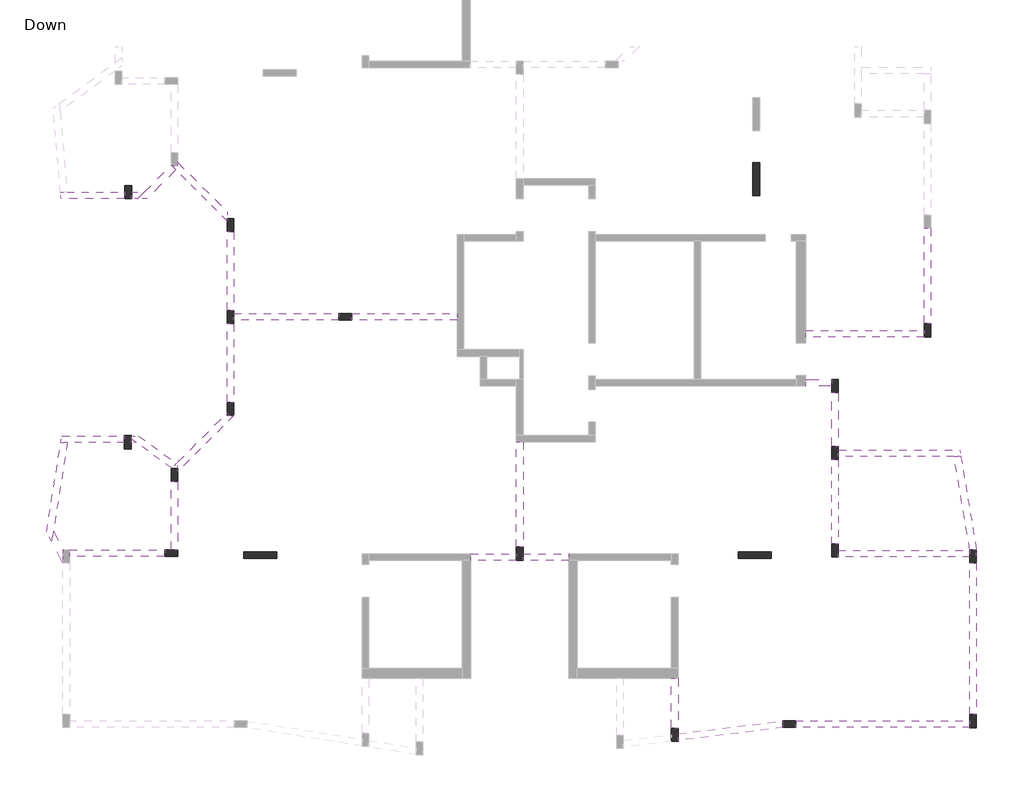
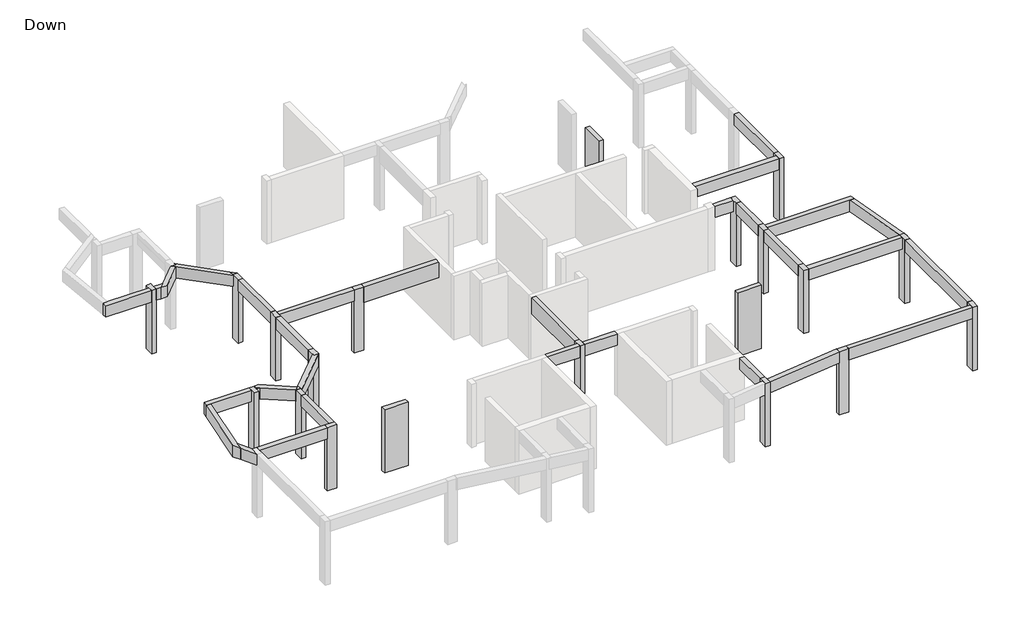
# One storey, part 2 of 3: 31 beams, 20 columns.
"""IFC4 building model written with IfcOpenShell, lengths in millimetres."""

from ifc_helpers import new_model, si_unit, frame, origin, origin_with_axes, place, context, project, spatial, polyline, outline, extrude, faceted_brep, element, save

model = new_model("IFC4")

# Units and contexts
model_context = context("Model", 3, world=origin())
ifc_project = project(units=[si_unit("LENGTHUNIT", "METRE", prefix="MILLI")], contexts=[model_context])

# Site, building, storey
site = spatial("IfcSite", under=ifc_project)
building = spatial("IfcBuilding", under=site)
storey = spatial("IfcBuildingStorey", under=building, Name="Down", Elevation=0.0)

# Beams
placement = place(None, origin())
element("IfcBeam", 1, ObjectType="Concrete Rectengular Beam : 20/50", at=placement, inside=storey, context=model_context, shape_type="Brep", body=[
    faceted_brep([(-18379.347479, -11765.3513235, 2850.0), (-18379.347479, -11965.3513235, 2850.0), (-15486.5645409, -11965.3513235, 2850.0), (-15486.5645409, -11765.3513235, 2850.0), (-18379.347479, -11965.3513235, 2650.0), (-18379.347479, -11965.3513235, 2350.0), (-15486.5645409, -11965.3513235, 2350.0), (-15486.5645409, -11965.3513235, 2650.0), (-18379.347479, -11765.3513235, 2350.0), (-15486.5645409, -11765.3513235, 2350.0)], [[[0, 1, 2, 3]], [[2, 1, 4, 5, 6, 7]], [[5, 8, 9, 6]], [[8, 0, 3, 9]], [[1, 0, 8, 5, 4]], [[3, 2, 7, 6, 9]]]),
])
element("IfcBeam", 2, ObjectType="Concrete Rectengular Beam : 20/50", at=placement, inside=storey, context=model_context, shape_type="Brep", body=[
    faceted_brep([(-15286.5645409, -9691.9014804, 2850.0), (-15286.5645409, -11765.3513235, 2850.0), (-15089.2187138, -11765.3513235, 2850.0), (-15089.2187138, -9691.9014804, 2850.0), (-15286.5645409, -11765.3513235, 2350.0), (-15286.5645409, -11765.3513235, 2650.0), (-15286.5645409, -9691.9014804, 2350.0), (-15086.5645409, -9691.9014804, 2350.0), (-15086.5645409, -11765.3513235, 2350.0), (-15086.5645409, -9691.9014804, 2650.0), (-15086.5645409, -11765.3513235, 2650.0), (-15089.2187138, -9691.9014804, 2650.0), (-15089.2187138, -11765.3513235, 2650.0)], [[[0, 1, 2, 3]], [[4, 5, 1, 0, 6]], [[6, 7, 8, 4]], [[8, 7, 9, 10]], [[7, 6, 0, 3, 11, 9]], [[1, 5, 4, 8, 10, 12, 2]], [[11, 12, 10, 9]], [[12, 11, 3, 2]]]),
    faceted_brep([(-15086.5645409, -9098.1046694, 2850.0), (-15086.5645409, -9098.1046694, 2350.0), (-15129.6352736, -9141.1754021, 2350.0), (-15272.8194649, -9284.3595934, 2350.0), (-15280.3613519, -9291.9014804, 2350.0), (-15280.3613519, -9291.9014804, 2850.0), (-15272.8194649, -9284.3595934, 2850.0), (-15129.6352736, -9141.1754021, 2850.0), (-15086.5645409, -9291.9014804, 2850.0), (-15086.5645409, -9291.9014804, 2350.0)], [[[0, 1, 2, 3, 4, 5, 6, 7]], [[8, 5, 4, 9]], [[5, 8, 0, 7, 6]], [[9, 4, 3, 2, 1]], [[1, 0, 8, 9]]]),
])
element("IfcBeam", 3, ObjectType="Concrete Rectengular Beam : 20/50", at=placement, inside=storey, context=model_context, shape_type="Brep", body=[
    faceted_brep([(-13387.4363964, -7681.8192373, 2850.0), (-13587.4363964, -7681.8192373, 2850.0), (-13587.4363964, -7598.9765249, 2850.0), (-15086.5645409, -9098.1046694, 2850.0), (-15086.5645409, -9291.9014804, 2850.0), (-15086.5645409, -9380.9473819, 2850.0), (-15086.5645409, -9380.9473819, 2650.0), (-15086.5645409, -9380.9473819, 2350.0), (-13387.4363964, -7681.8192373, 2350.0), (-13387.4363964, -7681.8192373, 2650.0), (-13587.4363964, -7681.8192373, 2350.0), (-15086.5645409, -9291.9014804, 2350.0), (-15086.5645409, -9098.1046694, 2350.0), (-13587.4363964, -7598.9765249, 2350.0)], [[[0, 1, 2, 3, 4, 5]], [[0, 5, 6, 7, 8, 9]], [[10, 8, 7, 11, 12, 13]], [[2, 13, 12, 3]], [[10, 1, 0, 9, 8]], [[1, 10, 13, 2]], [[3, 12, 11, 7, 6, 5, 4]]]),
])
element("IfcBeam", 4, ObjectType="Concrete Rectengular Beam : 20/50", at=placement, inside=storey, context=model_context, shape_type="Brep", body=[
    faceted_brep([(-15272.8194649, -9284.3595934, 2850.0), (-15129.6352736, -9141.1754021, 2850.0), (-16288.4232212, -8299.2666773, 2850.0), (-16461.5111803, -8299.2666773, 2850.0), (-16508.8112897, -8364.3696928, 2850.0), (-16508.8112897, -8386.3589683, 2850.0), (-16353.4071605, -8499.2666773, 2850.0), (-15286.5645409, -9274.373211, 2850.0), (-15129.6352736, -9141.1754021, 2350.0), (-16288.4232212, -8299.2666773, 2350.0), (-15272.8194649, -9284.3595934, 2350.0), (-16353.4071605, -8499.2666773, 2350.0), (-16508.8112897, -8386.3589683, 2350.0), (-16508.8112897, -8364.3696928, 2350.0), (-16461.5111803, -8299.2666773, 2350.0)], [[[0, 1, 2, 3, 4, 5, 6, 7]], [[1, 8, 9, 2]], [[8, 10, 11, 12, 13, 14, 9]], [[5, 12, 11, 10, 0, 7, 6]], [[1, 0, 10, 8]], [[3, 14, 13, 4]], [[3, 2, 9, 14]], [[5, 4, 13, 12]]]),
])
element("IfcBeam", 5, ObjectType="Concrete Rectengular Beam : 20/50", at=placement, inside=storey, context=model_context, shape_type="Brep", body=[
    faceted_brep([(-16508.8112897, -8386.3589683, 2850.0), (-16508.8112897, -8499.2666773, 2850.0), (-16353.4071605, -8499.2666773, 2850.0), (-16508.8112897, -8499.2666773, 2650.0), (-16508.8112897, -8499.2666773, 2350.0), (-16353.4071605, -8499.2666773, 2350.0), (-16353.4071605, -8499.2666773, 2650.0), (-16508.8112897, -8386.3589683, 2350.0)], [[[0, 1, 2]], [[1, 3, 4, 5, 6, 2]], [[4, 3, 1, 0, 7]], [[0, 2, 6, 5, 7]], [[4, 7, 5]]]),
    faceted_brep([(-16508.8112897, -8299.2666773, 2350.0), (-16508.8112897, -8299.2666773, 2850.0), (-16461.5111803, -8299.2666773, 2850.0), (-16461.5111803, -8299.2666773, 2350.0), (-16508.8112897, -8364.3696928, 2350.0), (-16508.8112897, -8364.3696928, 2850.0)], [[[0, 1, 2, 3]], [[4, 0, 3]], [[2, 5, 4, 3]], [[1, 5, 2]], [[1, 0, 4, 5]]]),
])
element("IfcBeam", 6, ObjectType="Concrete Rectengular Beam : 20/50", at=placement, inside=storey, context=model_context, shape_type="Brep", body=[
    faceted_brep([(-16708.8112897, -8499.2666773, 2850.0), (-16708.8112897, -8299.2666773, 2850.0), (-18614.2193583, -8299.2666773, 2850.0), (-18645.8962463, -8499.2666773, 2850.0), (-18443.4032212, -8499.2666773, 2850.0), (-16708.8112897, -8299.2666773, 2350.0), (-18614.2193583, -8299.2666773, 2350.0), (-16708.8112897, -8499.2666773, 2350.0), (-18443.4032212, -8499.2666773, 2350.0), (-18645.8962463, -8499.2666773, 2350.0), (-16708.8112897, -8499.2666773, 2650.0)], [[[0, 1, 2, 3, 4]], [[1, 5, 6, 2]], [[5, 7, 8, 9, 6]], [[7, 10, 0, 4, 3, 9, 8]], [[1, 0, 10, 7, 5]], [[3, 2, 6, 9]]]),
])
element("IfcBeam", 7, ObjectType="Concrete Rectengular Beam : 20/50", at=placement, inside=storey, context=model_context, shape_type="Brep", body=[
    faceted_brep([(-18443.4032212, -8499.2666773, 2850.0), (-18645.8962463, -8499.2666773, 2850.0), (-19077.0882285, -11221.7057077, 2850.0), (-18921.0696697, -11515.1339402, 2850.0), (-18869.0821124, -11186.8974215, 2850.0), (-18645.8962463, -8499.2666773, 2350.0), (-19077.0882285, -11221.7057077, 2350.0), (-18443.4032212, -8499.2666773, 2350.0), (-18869.0821124, -11186.8974215, 2350.0), (-18921.0696697, -11515.1339402, 2350.0), (-18443.4032212, -8499.2666773, 2650.0)], [[[0, 1, 2, 3, 4]], [[1, 5, 6, 2]], [[5, 7, 8, 9, 6]], [[3, 9, 8, 7, 10, 0, 4]], [[1, 0, 10, 7, 5]], [[3, 2, 6, 9]]]),
])
element("IfcBeam", 8, ObjectType="Concrete Rectengular Beam : 20/50", at=placement, inside=storey, context=model_context, shape_type="Brep", body=[
    faceted_brep([(-18869.0821124, -11186.8974215, 2850.0), (-18561.5127169, -11765.3513235, 2850.0), (-18561.5127169, -11765.3513235, 2650.0), (-18561.5127169, -11765.3513235, 2350.0), (-18869.0821124, -11186.8974215, 2350.0), (-18869.0821124, -11186.8974215, 2650.0), (-18921.0696697, -11515.1339402, 2850.0), (-18921.0696697, -11515.1339402, 2350.0), (-18579.347479, -11765.3513235, 2350.0), (-18579.347479, -11765.3513235, 2850.0), (-18579.347479, -11965.3513235, 2850.0), (-18579.347479, -12157.819908, 2850.0), (-18579.347479, -12157.819908, 2350.0), (-18579.347479, -11965.3513235, 2350.0)], [[[0, 1, 2, 3, 4, 5]], [[6, 0, 5, 4, 7]], [[8, 9, 10, 11, 12, 13]], [[9, 8, 3, 2, 1]], [[0, 6, 11, 10, 9, 1]], [[6, 7, 12, 11]], [[7, 4, 3, 8, 13, 12]]]),
])
element("IfcBeam", 9, ObjectType="Concrete Rectengular Beam : 20/50", at=placement, inside=storey, context=model_context, shape_type="Brep", body=[
    faceted_brep([(-13387.4363964, -4887.4320305, 2850.0), (-13587.4363964, -4887.4320305, 2850.0), (-13587.4363964, -7281.8192373, 2850.0), (-13387.4363964, -7281.8192373, 2850.0), (-13387.4363964, -7281.8192373, 2650.0), (-13387.4363964, -7281.8192373, 2350.0), (-13387.4363964, -4887.4320305, 2350.0), (-13387.4363964, -4887.4320305, 2650.0), (-13587.4363964, -4887.4320305, 2350.0), (-13587.4363964, -7281.8192373, 2350.0)], [[[0, 1, 2, 3]], [[0, 3, 4, 5, 6, 7]], [[8, 6, 5, 9]], [[1, 8, 9, 2]], [[1, 0, 7, 6, 8]], [[3, 2, 9, 5, 4]]]),
])
element("IfcBeam", 10, ObjectType="Concrete Rectengular Beam : 20/50", at=placement, inside=storey, context=model_context, shape_type="Brep", body=[
    faceted_brep([(-13387.4363964, -4587.4320305, 2850.0), (-13387.4363964, -4787.4320305, 2850.0), (-10195.9008278, -4787.4320305, 2850.0), (-10195.9008278, -4587.4320305, 2850.0), (-13387.4363964, -4787.4320305, 2650.0), (-13387.4363964, -4787.4320305, 2350.0), (-10195.9008278, -4787.4320305, 2350.0), (-13387.4363964, -4587.4320305, 2350.0), (-10195.9008278, -4587.4320305, 2350.0), (-13387.4363964, -4587.4320305, 2650.0)], [[[0, 1, 2, 3]], [[1, 4, 5, 6, 2]], [[5, 7, 8, 6]], [[7, 9, 0, 3, 8]], [[5, 4, 1, 0, 9, 7]], [[3, 2, 6, 8]]]),
])
element("IfcBeam", 11, ObjectType="Concrete Rectengular Beam : 20/50", at=placement, inside=storey, context=model_context, shape_type="Brep", body=[
    faceted_brep([(-13387.4363964, -2088.5879682, 2850.0), (-13587.4363964, -2088.5879682, 2850.0), (-13587.4363964, -4487.4320305, 2850.0), (-13387.4363964, -4487.4320305, 2850.0), (-13387.4363964, -4487.4320305, 2650.0), (-13387.4363964, -4487.4320305, 2350.0), (-13387.4363964, -2088.5879682, 2350.0), (-13387.4363964, -2088.5879682, 2650.0), (-13587.4363964, -2088.5879682, 2350.0), (-13587.4363964, -4487.4320305, 2350.0)], [[[0, 1, 2, 3]], [[0, 3, 4, 5, 6, 7]], [[8, 6, 5, 9]], [[1, 8, 9, 2]], [[1, 0, 7, 6, 8]], [[3, 2, 9, 5, 4]]]),
    faceted_brep([(-13387.4363964, -1685.7442295, 2350.0), (-13587.4363964, -1485.8326961, 2350.0), (-13587.4363964, -1485.8326961, 2650.0), (-13387.4363964, -1685.7442295, 2650.0), (-13587.4363964, -1688.5879682, 2350.0), (-13387.4363964, -1688.5879682, 2350.0), (-13387.4363964, -1688.5879682, 2650.0), (-13388.8740156, -1688.5879682, 2650.0), (-13388.8740156, -1688.5879682, 2850.0), (-13587.4363964, -1688.5879682, 2850.0), (-13587.4363964, -1490.0255874, 2850.0), (-13587.4363964, -1490.0255874, 2650.0)], [[[0, 1, 2, 3]], [[4, 5, 6, 7, 8, 9]], [[10, 9, 8]], [[5, 0, 3, 6]], [[1, 0, 5, 4]], [[1, 4, 9, 10, 11, 2]], [[11, 7, 6, 3, 2]], [[7, 11, 10, 8]]]),
])
element("IfcBeam", 12, ObjectType="Concrete Rectengular Beam : 20/50", at=placement, inside=storey, context=model_context, shape_type="Brep", body=[
    faceted_brep([(-15089.2187138, -83.5414212, 2850.0), (-15273.253528, -83.5414212, 2850.0), (-13587.4363964, -1768.6128602, 2850.0), (-13587.4363964, -1688.5879682, 2850.0), (-13587.4363964, -1490.0255874, 2850.0), (-15089.2187138, 11.75673, 2850.0), (-13587.4363964, -1485.8326961, 2350.0), (-15089.2187138, 15.2853334, 2350.0), (-15089.2187138, 15.2853334, 2650.0), (-13587.4363964, -1485.8326961, 2650.0), (-15089.2187138, -83.5414212, 2350.0), (-13587.4363964, -1688.5879682, 2350.0), (-13587.4363964, -1768.6128602, 2350.0), (-15144.8886874, -211.8494818, 2350.0), (-15273.253528, -83.5414212, 2350.0), (-15089.2187138, 11.75673, 2650.0), (-13587.4363964, -1490.0255874, 2650.0)], [[[0, 1, 2, 3, 4, 5]], [[6, 7, 8, 9]], [[10, 7, 6, 11, 12, 13, 14]], [[1, 14, 13, 12, 2]], [[10, 0, 5, 15, 8, 7]], [[0, 10, 14, 1]], [[12, 11, 6, 9, 16, 4, 3, 2]], [[15, 16, 9, 8]], [[16, 15, 5, 4]]]),
])
element("IfcBeam", 13, ObjectType="Concrete Rectengular Beam : 20/50", at=placement, inside=storey, context=model_context, shape_type="Brep", body=[
    faceted_brep([(-16307.2350357, -1091.3531176, 2850.0), (-16024.3923233, -1091.3531176, 2850.0), (-15144.8886874, -211.8494818, 2850.0), (-15273.253528, -83.5414212, 2850.0), (-15289.2187138, -83.5414212, 2850.0), (-15289.2187138, -73.3367957, 2850.0), (-16107.2350357, -891.3531176, 2850.0), (-16307.2350357, -1091.3531176, 2350.0), (-15289.2187138, -73.3367957, 2650.0), (-15289.2187138, -73.3367957, 2350.0), (-16107.2350357, -891.3531176, 2350.0), (-16024.3923233, -1091.3531176, 2350.0), (-15289.2187138, -83.5414212, 2350.0), (-15273.253528, -83.5414212, 2350.0), (-15144.8886874, -211.8494818, 2350.0)], [[[0, 1, 2, 3, 4, 5, 6]], [[7, 0, 6, 5, 8, 9, 10]], [[11, 7, 10, 9, 12, 13, 14]], [[1, 11, 14, 2]], [[1, 0, 7, 11]], [[2, 14, 13, 3]], [[4, 12, 9, 8, 5]], [[12, 4, 3, 13]]]),
])
element("IfcBeam", 14, ObjectType="Concrete Rectengular Beam : 20/50", at=placement, inside=storey, context=model_context, shape_type="Brep", body=[
    faceted_brep([(-16494.0770885, -891.3531176, 2850.0), (-16494.0770885, -1091.3531176, 2850.0), (-16307.2350357, -1091.3531176, 2850.0), (-16107.2350357, -891.3531176, 2850.0), (-16494.0770885, -891.3531176, 2350.0), (-16494.0770885, -891.3531176, 2650.0), (-16107.2350357, -891.3531176, 2650.0), (-16107.2350357, -891.3531176, 2350.0), (-16494.0770885, -1091.3531176, 2350.0), (-16307.2350357, -1091.3531176, 2350.0)], [[[0, 1, 2, 3]], [[4, 5, 0, 3, 6, 7]], [[8, 4, 7, 9]], [[9, 2, 1, 8]], [[1, 0, 5, 4, 8]], [[3, 2, 9, 7, 6]]]),
])
element("IfcBeam", 15, ObjectType="Concrete Rectengular Beam : 20/50", at=placement, inside=storey, context=model_context, shape_type="Brep", body=[
    faceted_brep([(-16694.0770885, -1091.3531176, 2850.0), (-16694.0770885, -891.3531176, 2850.0), (-18452.5305511, -891.3531176, 2850.0), (-18653.293728, -891.3531176, 2850.0), (-18635.8050681, -1091.3531176, 2850.0), (-16694.0770885, -891.3531176, 2650.0), (-16694.0770885, -891.3531176, 2350.0), (-18452.5305511, -891.3531176, 2350.0), (-18653.293728, -891.3531176, 2350.0), (-16694.0770885, -1091.3531176, 2350.0), (-18635.8050681, -1091.3531176, 2350.0)], [[[0, 1, 2, 3, 4]], [[1, 5, 6, 7, 8, 3, 2]], [[6, 9, 10, 8, 7]], [[4, 10, 9, 0]], [[1, 0, 9, 6, 5]], [[4, 3, 8, 10]]]),
])
element("IfcBeam", 16, ObjectType="Concrete Rectengular Beam : 20/50", at=placement, inside=storey, context=model_context, shape_type="SweptSolid", body=[
    extrude(outline(polyline([(7791.3944084, -4891.9879156), (7591.3944084, -4891.9879156), (7591.3944084, -1988.6737606), (7791.3944084, -1988.6737606), (7791.3944084, -4891.9879156)])), frame((0.0, 0.0, 2350.0), z_axis=(0.0, 0.0, 1.0), x_axis=(1.0, 0.0, 0.0)), (0.0, 0.0, 1.0), 500.0),
])
element("IfcBeam", 17, ObjectType="Concrete Rectengular Beam : 20/50", at=placement, inside=storey, context=model_context, shape_type="Brep", body=[
    faceted_brep([(7591.3944084, -5291.9879156, 2850.0), (7591.3944084, -5091.9879156, 2850.0), (3996.1514357, -5091.9879156, 2850.0), (3996.1514357, -5291.9879156, 2850.0), (7591.3944084, -5091.9879156, 2650.0), (7591.3944084, -5091.9879156, 2350.0), (3996.1514357, -5091.9879156, 2350.0), (3996.1514357, -5091.9879156, 2650.0), (7591.3944084, -5291.9879156, 2350.0), (3996.1514357, -5291.9879156, 2350.0)], [[[0, 1, 2, 3]], [[1, 4, 5, 6, 7, 2]], [[5, 8, 9, 6]], [[8, 0, 3, 9]], [[1, 0, 8, 5, 4]], [[3, 2, 7, 6, 9]]]),
])
element("IfcBeam", 18, ObjectType="Concrete Rectengular Beam : 20/50", at=placement, inside=storey, context=model_context, shape_type="Brep", body=[
    faceted_brep([(4785.5431075, -6790.494584, 2850.0), (4785.5431075, -6590.494584, 2850.0), (3996.1514357, -6590.494584, 2850.0), (3996.1514357, -6790.494584, 2850.0), (4785.5431075, -6590.494584, 2350.0), (3996.1514357, -6590.494584, 2350.0), (4785.5431075, -6790.494584, 2350.0), (3996.1514357, -6790.494584, 2350.0), (4785.5431075, -6790.494584, 2650.0)], [[[0, 1, 2, 3]], [[1, 4, 5, 2]], [[4, 6, 7, 5]], [[6, 8, 0, 3, 7]], [[1, 0, 8, 6, 4]], [[3, 2, 5, 7]]]),
])
element("IfcBeam", 19, ObjectType="Concrete Rectengular Beam : 20/50", at=placement, inside=storey, context=model_context, shape_type="Brep", body=[
    faceted_brep([(4785.5431075, -8626.3350173, 2850.0), (4985.5431075, -8626.3350173, 2850.0), (4985.5431075, -6990.494584, 2850.0), (4785.5431075, -6990.494584, 2850.0), (4785.5431075, -6990.494584, 2650.0), (4785.5431075, -6990.494584, 2350.0), (4785.5431075, -8626.3350173, 2350.0), (4785.5431075, -8626.3350173, 2650.0), (4985.5431075, -8626.3350173, 2350.0), (4985.5431075, -6990.494584, 2350.0)], [[[0, 1, 2, 3]], [[0, 3, 4, 5, 6, 7]], [[8, 6, 5, 9]], [[1, 8, 9, 2]], [[1, 0, 7, 6, 8]], [[3, 2, 9, 5, 4]]]),
])
element("IfcBeam", 20, ObjectType="Concrete Rectengular Beam : 20/50", at=placement, inside=storey, context=model_context, shape_type="Brep", body=[
    faceted_brep([(4985.5431075, -8726.3350173, 2850.0), (4985.5431075, -8926.3350173, 2850.0), (8500.876934, -8926.3350173, 2850.0), (8703.6540317, -8926.3350173, 2850.0), (8670.2092809, -8726.3350173, 2850.0), (4985.5431075, -8926.3350173, 2650.0), (4985.5431075, -8926.3350173, 2350.0), (8500.876934, -8926.3350173, 2350.0), (8703.6540317, -8926.3350173, 2350.0), (4985.5431075, -8726.3350173, 2350.0), (8670.2092809, -8726.3350173, 2350.0)], [[[0, 1, 2, 3, 4]], [[1, 5, 6, 7, 8, 3, 2]], [[6, 9, 10, 8, 7]], [[9, 0, 4, 10]], [[0, 9, 6, 5, 1]], [[4, 3, 8, 10]]]),
])
element("IfcBeam", 21, ObjectType="Concrete Rectengular Beam : 20/50", at=placement, inside=storey, context=model_context, shape_type="Brep", body=[
    faceted_brep([(8977.0164469, -11773.6548619, 2850.0), (8977.0164469, -11765.3513235, 2850.0), (9177.0164469, -11765.3513235, 2850.0), (9177.0164469, -11955.7089512, 2850.0), (9209.3336029, -11950.304755, 2850.0), (8703.6540317, -8926.3350173, 2850.0), (8500.876934, -8926.3350173, 2850.0), (8500.876934, -8926.3350173, 2650.0), (8500.876934, -8926.3350173, 2350.0), (8977.0164469, -11773.6548619, 2350.0), (8977.0164469, -11773.6548619, 2650.0), (8977.0164469, -11765.3513235, 2350.0), (8703.6540317, -8926.3350173, 2350.0), (9209.3336029, -11950.304755, 2350.0), (9177.0164469, -11955.7089512, 2350.0), (9177.0164469, -11765.3513235, 2350.0)], [[[0, 1, 2, 3, 4, 5, 6]], [[0, 6, 7, 8, 9, 10]], [[11, 9, 8, 12, 13, 14, 15]], [[5, 4, 13, 12]], [[11, 1, 0, 10, 9]], [[1, 11, 15, 2]], [[6, 5, 12, 8, 7]], [[13, 4, 3, 14]], [[2, 15, 14, 3]]]),
])
element("IfcBeam", 22, ObjectType="Concrete Rectengular Beam : 20/50", at=placement, inside=storey, context=model_context, shape_type="Brep", body=[
    faceted_brep([(4985.5431075, -11983.2914692, 2350.0), (8977.0164469, -11983.2914692, 2350.0), (8977.0164469, -11983.2914692, 2650.0), (8977.0164469, -11983.2914692, 2850.0), (4985.5431075, -11983.2914692, 2850.0), (4985.5431075, -11983.2914692, 2650.0), (8977.0164469, -11783.2914692, 2850.0), (8977.0164469, -11783.2914692, 2350.0), (8977.0164469, -11783.2914692, 2650.0), (4985.5431075, -11783.2914692, 2850.0), (4985.5431075, -11783.2914692, 2650.0), (4985.5431075, -11783.2914692, 2350.0)], [[[0, 1, 2, 3, 4, 5]], [[6, 3, 2, 1, 7, 8]], [[4, 9, 10, 11, 0, 5]], [[3, 6, 9, 4]], [[6, 8, 7, 11, 10, 9]], [[7, 1, 0, 11]]]),
])
element("IfcBeam", 23, ObjectType="Concrete Rectengular Beam : 20/50", at=placement, inside=storey, context=model_context, shape_type="Brep", body=[
    faceted_brep([(4785.5431075, -11583.2914692, 2850.0), (4985.5431075, -11583.2914692, 2850.0), (4985.5431075, -9026.3350173, 2850.0), (4785.5431075, -9026.3350173, 2850.0), (4985.5431075, -11583.2914692, 2350.0), (4985.5431075, -9026.3350173, 2350.0), (4785.5431075, -11583.2914692, 2350.0), (4785.5431075, -9026.3350173, 2350.0), (4785.5431075, -9026.3350173, 2650.0), (4785.5431075, -11583.2914692, 2650.0)], [[[0, 1, 2, 3]], [[1, 4, 5, 2]], [[4, 6, 7, 5]], [[0, 3, 8, 7, 6, 9]], [[1, 0, 9, 6, 4]], [[3, 2, 5, 7, 8]]]),
])
element("IfcBeam", 24, ObjectType="Concrete Rectengular Beam : 20/50", at=placement, inside=storey, context=model_context, shape_type="SweptSolid", body=[
    extrude(outline(polyline([(9177.0164469, -16771.5953491), (8977.0164469, -16771.5953491), (8977.0164469, -12165.3513235), (9177.0164469, -12165.3513235), (9177.0164469, -16771.5953491)])), frame((0.0, 0.0, 2350.0), z_axis=(0.0, 0.0, 1.0), x_axis=(1.0, 0.0, 0.0)), (0.0, 0.0, 1.0), 500.0),
])
element("IfcBeam", 25, ObjectType="Concrete Rectengular Beam : 20/50", at=placement, inside=storey, context=model_context, shape_type="Brep", body=[
    faceted_brep([(3695.6052151, -16969.7313812, 2850.0), (3695.6052151, -17169.7313812, 2850.0), (8977.0164469, -17169.7313812, 2850.0), (8977.0164469, -16969.7313812, 2850.0), (8977.0164469, -16969.7313812, 2650.0), (8977.0164469, -16969.7313812, 2350.0), (3695.6052151, -16969.7313812, 2350.0), (3695.6052151, -16969.7313812, 2650.0), (3695.6052151, -17169.7313812, 2350.0), (8977.0164469, -17169.7313812, 2350.0)], [[[0, 1, 2, 3]], [[0, 3, 4, 5, 6, 7]], [[8, 6, 5, 9]], [[1, 8, 9, 2]], [[1, 0, 7, 6, 8]], [[2, 9, 5, 4, 3]]]),
    faceted_brep([(3295.6052151, -17069.7313812, 2850.0), (3289.488953, -16969.7313812, 2850.0), (3289.488953, -16969.7313812, 2650.0), (3289.488953, -16969.7313812, 2350.0), (3295.6052151, -17069.7313812, 2350.0), (3295.6052151, -16969.7313812, 2850.0), (3295.6052151, -16969.7313812, 2350.0), (3295.6052151, -16969.7313812, 2650.0)], [[[0, 1, 2, 3, 4]], [[5, 0, 4, 6, 7]], [[1, 0, 5]], [[1, 5, 7, 6, 3, 2]], [[4, 3, 6]]]),
])
element("IfcBeam", 26, ObjectType="Concrete Rectengular Beam : 20/50", at=placement, inside=storey, context=model_context, shape_type="Brep", body=[
    faceted_brep([(112.3964523, -17561.3312539, 2850.0), (3301.7214771, -17169.7313812, 2850.0), (3295.6052151, -17169.7313812, 2850.0), (3295.6052151, -17069.7313812, 2850.0), (3289.488953, -16969.7313812, 2850.0), (112.3964523, -17359.8292888, 2850.0), (3289.488953, -16969.7313812, 2650.0), (3289.488953, -16969.7313812, 2350.0), (112.3964523, -17359.8292888, 2350.0), (112.3964523, -17359.8292888, 2650.0), (3295.6052151, -17069.7313812, 2350.0), (3295.6052151, -17169.7313812, 2350.0), (3301.7214771, -17169.7313812, 2350.0), (112.3964523, -17561.3312539, 2350.0)], [[[0, 1, 2, 3, 4, 5]], [[5, 4, 6, 7, 8, 9]], [[8, 7, 10, 11, 12, 13]], [[1, 0, 13, 12]], [[4, 3, 10, 7, 6]], [[0, 5, 9, 8, 13]], [[11, 2, 1, 12]], [[2, 11, 10, 3]]]),
])
element("IfcBeam", 27, ObjectType="Concrete Rectengular Beam : 20/50", at=placement, inside=storey, context=model_context, shape_type="Brep", body=[
    faceted_brep([(-87.6035477, -17190.4678354, 2850.0), (112.3964523, -17190.4678354, 2850.0), (112.3964523, -15667.9244771, 2850.0), (-87.6035477, -15667.9244771, 2850.0), (112.3964523, -17190.4678354, 2650.0), (112.3964523, -17190.4678354, 2350.0), (112.3964523, -15667.9244771, 2350.0), (112.3964523, -15667.9244771, 2650.0), (-87.6035477, -17190.4678354, 2350.0), (-87.6035477, -15667.9244771, 2350.0), (-87.6035477, -15667.9244771, 2650.0)], [[[0, 1, 2, 3]], [[2, 1, 4, 5, 6, 7]], [[5, 8, 9, 6]], [[8, 0, 3, 10, 9]], [[1, 0, 8, 5, 4]], [[3, 2, 7, 6, 9, 10]]]),
])
element("IfcBeam", 28, ObjectType="Concrete Rectengular Beam : 20/50", at=placement, inside=storey, context=model_context, shape_type="Brep", body=[
    faceted_brep([(-4597.6379386, -11883.2914692, 2850.0), (-4597.6379386, -12083.2914692, 2850.0), (-3204.5902544, -12083.2914692, 2850.0), (-3204.5902544, -11883.2914692, 2850.0), (-3204.5902544, -11883.2914692, 2650.0), (-3204.5902544, -11883.2914692, 2350.0), (-4597.6379386, -11883.2914692, 2350.0), (-4597.6379386, -11883.2914692, 2650.0), (-4597.6379386, -12083.2914692, 2350.0), (-3204.5902544, -12083.2914692, 2350.0)], [[[0, 1, 2, 3]], [[0, 3, 4, 5, 6, 7]], [[8, 6, 5, 9]], [[1, 8, 9, 2]], [[1, 0, 7, 6, 8]], [[3, 2, 9, 5, 4]]]),
])
element("IfcBeam", 29, ObjectType="Concrete Rectengular Beam : 20/50", at=placement, inside=storey, context=model_context, shape_type="Brep", body=[
    faceted_brep([(-4797.6379386, -12083.2914692, 2850.0), (-4797.6379386, -11883.2914692, 2850.0), (-6190.6856227, -11883.2914692, 2850.0), (-6190.6856227, -12083.2914692, 2850.0), (-4797.6379386, -11883.2914692, 2650.0), (-4797.6379386, -11883.2914692, 2350.0), (-6190.6856227, -11883.2914692, 2350.0), (-6190.6856227, -11883.2914692, 2650.0), (-4797.6379386, -12083.2914692, 2350.0), (-6190.6856227, -12083.2914692, 2350.0)], [[[0, 1, 2, 3]], [[2, 1, 4, 5, 6, 7]], [[5, 8, 9, 6]], [[8, 0, 3, 9]], [[1, 0, 8, 5, 4]], [[3, 2, 7, 6, 9]]]),
])
element("IfcBeam", 30, ObjectType="Concrete Rectengular Beam : 20/70", at=placement, inside=storey, context=model_context, shape_type="Brep", body=[
    faceted_brep([(-9795.9008278, -4587.4320305, 2850.0), (-9795.9008278, -4787.4320305, 2850.0), (-6597.6379386, -4787.4320305, 2850.0), (-6597.6379386, -4587.4320305, 2850.0), (-9795.9008278, -4787.4320305, 2150.0), (-6597.6379386, -4787.4320305, 2150.0), (-6597.6379386, -4787.4320305, 2650.0), (-9795.9008278, -4587.4320305, 2150.0), (-6597.6379386, -4587.4320305, 2150.0), (-6597.6379386, -4587.4320305, 2650.0)], [[[0, 1, 2, 3]], [[1, 4, 5, 6, 2]], [[4, 7, 8, 5]], [[7, 0, 3, 9, 8]], [[1, 0, 7, 4]], [[3, 2, 6, 5, 8, 9]]]),
])
element("IfcBeam", 31, ObjectType="Concrete Rectengular Beam : 20/70", at=placement, inside=storey, context=model_context, shape_type="Brep", body=[
    faceted_brep([(-4797.6379386, -11683.2914692, 2850.0), (-4597.6379386, -11683.2914692, 2850.0), (-4597.6379386, -8483.2914692, 2850.0), (-4797.6379386, -8483.2914692, 2850.0), (-4597.6379386, -11683.2914692, 2150.0), (-4597.6379386, -8483.2914692, 2150.0), (-4597.6379386, -8483.2914692, 2650.0), (-4797.6379386, -11683.2914692, 2150.0), (-4797.6379386, -8483.2914692, 2150.0)], [[[0, 1, 2, 3]], [[1, 4, 5, 6, 2]], [[4, 7, 8, 5]], [[7, 0, 3, 8]], [[1, 0, 7, 4]], [[3, 2, 6, 5, 8]]]),
])

# Columns
element("IfcColumn", 32, ObjectType="Concrete Rectengular Column : 100/20", at=placement, inside=storey, context=model_context, shape_type="Brep", body=[
    faceted_brep([(-12084.0109343, -11824.8863444, 0.0), (-12084.0109343, -12024.8863444, 0.0), (-13084.0109343, -12024.8863444, 0.0), (-13084.0109343, -11824.8863444, 0.0), (-12084.0109343, -11824.8863444, 2850.0), (-12084.0109343, -12024.8863444, 2850.0), (-12084.0109343, -12024.8863444, 2650.0), (-12084.0109343, -11824.8863444, 2650.0), (-13084.0109343, -12024.8863444, 2850.0), (-13084.0109343, -12024.8863444, 2650.0), (-13084.0109343, -11824.8863444, 2850.0), (-13084.0109343, -11824.8863444, 2650.0)], [[[0, 1, 2, 3]], [[4, 5, 6, 1, 0, 7]], [[5, 8, 9, 2, 1, 6]], [[8, 10, 11, 3, 2, 9]], [[10, 4, 7, 0, 3, 11]], [[4, 10, 8, 5]]]),
])
element("IfcColumn", 33, ObjectType="Concrete Rectengular Column : 100/20", at=placement, inside=storey, context=model_context, shape_type="Brep", body=[
    faceted_brep([(2945.6091526, -11824.8863444, 0.0), (2945.6091526, -12024.8863444, 0.0), (1945.6091526, -12024.8863444, 0.0), (1945.6091526, -11824.8863444, 0.0), (2945.6091526, -11824.8863444, 2850.0), (2945.6091526, -12024.8863444, 2850.0), (2945.6091526, -12024.8863444, 2650.0), (2945.6091526, -11824.8863444, 2650.0), (1945.6091526, -12024.8863444, 2850.0), (1945.6091526, -12024.8863444, 2650.0), (1945.6091526, -11824.8863444, 2850.0), (1945.6091526, -11824.8863444, 2650.0)], [[[0, 1, 2, 3]], [[4, 5, 6, 1, 0, 7]], [[5, 8, 9, 2, 1, 6]], [[8, 10, 11, 3, 2, 9]], [[10, 4, 7, 0, 3, 11]], [[4, 10, 8, 5]]]),
])
element("IfcColumn", 34, ObjectType="Concrete Rectengular Column : 100/20", at=placement, inside=storey, context=model_context, shape_type="Brep", body=[
    faceted_brep([(2387.619868, 0.7719728, 0.0), (2587.619868, 0.7719728, 0.0), (2587.619868, -999.2280272, 0.0), (2387.619868, -999.2280272, 0.0), (2387.619868, 0.7719728, 2850.0), (2587.619868, 0.7719728, 2850.0), (2587.619868, 0.7719728, 2650.0), (2387.619868, 0.7719728, 2650.0), (2587.619868, -999.2280272, 2850.0), (2587.619868, -999.2280272, 2650.0), (2387.619868, -999.2280272, 2850.0), (2387.619868, -999.2280272, 2650.0)], [[[0, 1, 2, 3]], [[4, 5, 6, 1, 0, 7]], [[5, 8, 9, 2, 1, 6]], [[8, 10, 11, 3, 2, 9]], [[10, 4, 7, 0, 3, 11]], [[4, 10, 8, 5]]]),
])
element("IfcColumn", 35, ObjectType="Concrete Rectengular Column : 20/40", at=placement, inside=storey, context=model_context, shape_type="Brep", body=[
    faceted_brep([(-16694.0770885, -1091.3531176, 0.0), (-16694.0770885, -691.3531176, 0.0), (-16494.0770885, -691.3531176, 0.0), (-16494.0770885, -1091.3531176, 0.0), (-16694.0770885, -1091.3531176, 2850.0), (-16694.0770885, -891.3531176, 2850.0), (-16694.0770885, -691.3531176, 2850.0), (-16694.0770885, -691.3531176, 2650.0), (-16494.0770885, -691.3531176, 2850.0), (-16494.0770885, -691.3531176, 2650.0), (-16494.0770885, -891.3531176, 2850.0), (-16494.0770885, -1091.3531176, 2850.0)], [[[0, 1, 2, 3]], [[4, 5, 6, 7, 1, 0]], [[6, 8, 9, 2, 1, 7]], [[8, 10, 11, 3, 2, 9]], [[11, 4, 0, 3]], [[4, 11, 10, 8, 6, 5]]]),
])
element("IfcColumn", 36, ObjectType="Concrete Rectengular Column : 20/40", at=placement, inside=storey, context=model_context, shape_type="Brep", body=[
    faceted_brep([(-13387.4363964, -1688.5879682, 0.0), (-13387.4363964, -2088.5879682, 0.0), (-13587.4363964, -2088.5879682, 0.0), (-13587.4363964, -1688.5879682, 0.0), (-13387.4363964, -1688.5879682, 2850.0), (-13387.4363964, -2088.5879682, 2850.0), (-13387.4363964, -1688.5879682, 2650.0), (-13587.4363964, -2088.5879682, 2850.0), (-13587.4363964, -1688.5879682, 2850.0), (-13388.8740156, -1688.5879682, 2850.0)], [[[0, 1, 2, 3]], [[4, 5, 1, 0, 6]], [[5, 7, 2, 1]], [[7, 8, 3, 2]], [[8, 9, 4, 6, 0, 3]], [[4, 9, 8, 7, 5]]]),
])
element("IfcColumn", 37, ObjectType="Concrete Rectengular Column : 20/40", at=placement, inside=storey, context=model_context, shape_type="Brep", body=[
    faceted_brep([(-13387.4363964, -4487.4320305, 0.0), (-13387.4363964, -4887.4320305, 0.0), (-13587.4363964, -4887.4320305, 0.0), (-13587.4363964, -4487.4320305, 0.0), (-13387.4363964, -4487.4320305, 2850.0), (-13387.4363964, -4587.4320305, 2850.0), (-13387.4363964, -4787.4320305, 2850.0), (-13387.4363964, -4887.4320305, 2850.0), (-13587.4363964, -4887.4320305, 2850.0), (-13587.4363964, -4487.4320305, 2850.0)], [[[0, 1, 2, 3]], [[4, 5, 6, 7, 1, 0]], [[7, 8, 2, 1]], [[8, 9, 3, 2]], [[9, 4, 0, 3]], [[4, 9, 8, 7, 6, 5]]]),
])
element("IfcColumn", 38, ObjectType="Concrete Rectengular Column : 20/40", at=placement, inside=storey, context=model_context, shape_type="SweptSolid", body=[
    extrude(outline(polyline([(-13387.4363964, -7281.8192373), (-13387.4363964, -7681.8192373), (-13587.4363964, -7681.8192373), (-13587.4363964, -7281.8192373), (-13387.4363964, -7281.8192373)])), origin_with_axes(), (0.0, 0.0, 1.0), 2850.0),
])
element("IfcColumn", 39, ObjectType="Concrete Rectengular Column : 20/40", at=placement, inside=storey, context=model_context, shape_type="Brep", body=[
    faceted_brep([(-15086.5645409, -9291.9014804, 0.0), (-15086.5645409, -9691.9014804, 0.0), (-15286.5645409, -9691.9014804, 0.0), (-15286.5645409, -9291.9014804, 0.0), (-15086.5645409, -9291.9014804, 2850.0), (-15086.5645409, -9380.9473819, 2850.0), (-15086.5645409, -9691.9014804, 2850.0), (-15086.5645409, -9691.9014804, 2650.0), (-15089.2187138, -9691.9014804, 2850.0), (-15286.5645409, -9691.9014804, 2850.0), (-15286.5645409, -9291.9014804, 2850.0)], [[[0, 1, 2, 3]], [[4, 5, 6, 7, 1, 0]], [[6, 8, 9, 2, 1, 7]], [[9, 10, 3, 2]], [[10, 4, 0, 3]], [[4, 10, 9, 8, 6, 5]]]),
])
element("IfcColumn", 40, ObjectType="Concrete Rectengular Column : 20/40", at=placement, inside=storey, context=model_context, shape_type="Brep", body=[
    faceted_brep([(-16508.8112897, -8294.3603589, 0.0), (-16508.8112897, -8694.3603589, 0.0), (-16708.8112897, -8694.3603589, 0.0), (-16708.8112897, -8294.3603589, 0.0), (-16508.8112897, -8294.3603589, 2850.0), (-16508.8112897, -8364.3696928, 2850.0), (-16508.8112897, -8386.3589683, 2850.0), (-16508.8112897, -8499.2666773, 2850.0), (-16508.8112897, -8694.3603589, 2850.0), (-16508.8112897, -8694.3603589, 2650.0), (-16708.8112897, -8694.3603589, 2850.0), (-16708.8112897, -8694.3603589, 2650.0), (-16708.8112897, -8499.2666773, 2850.0), (-16708.8112897, -8294.3603589, 2850.0)], [[[0, 1, 2, 3]], [[4, 5, 6, 7, 8, 9, 1, 0]], [[8, 10, 11, 2, 1, 9]], [[10, 12, 13, 3, 2, 11]], [[13, 4, 0, 3]], [[4, 13, 12, 10, 8, 7, 6, 5]]]),
])
element("IfcColumn", 41, ObjectType="Concrete Rectengular Column : 20/40", at=placement, inside=storey, context=model_context, shape_type="Brep", body=[
    faceted_brep([(-15486.5645409, -11765.3513235, 0.0), (-15086.5645409, -11765.3513235, 0.0), (-15086.5645409, -11965.3513235, 0.0), (-15486.5645409, -11965.3513235, 0.0), (-15486.5645409, -11765.3513235, 2850.0), (-15286.5645409, -11765.3513235, 2850.0), (-15089.2187138, -11765.3513235, 2850.0), (-15086.5645409, -11765.3513235, 2850.0), (-15086.5645409, -11765.3513235, 2650.0), (-15086.5645409, -11965.3513235, 2850.0), (-15086.5645409, -11965.3513235, 2650.0), (-15486.5645409, -11965.3513235, 2850.0)], [[[0, 1, 2, 3]], [[4, 5, 6, 7, 8, 1, 0]], [[7, 9, 10, 2, 1, 8]], [[9, 11, 3, 2, 10]], [[11, 4, 0, 3]], [[4, 11, 9, 7, 6, 5]]]),
])
element("IfcColumn", 42, ObjectType="Concrete Rectengular Column : 20/40", at=placement, inside=storey, context=model_context, shape_type="Brep", body=[
    faceted_brep([(-4597.6379386, -11683.2914692, 0.0), (-4597.6379386, -12083.2914692, 0.0), (-4797.6379386, -12083.2914692, 0.0), (-4797.6379386, -11683.2914692, 0.0), (-4597.6379386, -11683.2914692, 2850.0), (-4597.6379386, -11883.2914692, 2850.0), (-4597.6379386, -12083.2914692, 2850.0), (-4797.6379386, -12083.2914692, 2850.0), (-4797.6379386, -11883.2914692, 2850.0), (-4797.6379386, -11683.2914692, 2850.0)], [[[0, 1, 2, 3]], [[4, 5, 6, 1, 0]], [[6, 7, 2, 1]], [[7, 8, 9, 3, 2]], [[9, 4, 0, 3]], [[4, 9, 8, 7, 6, 5]]]),
])
element("IfcColumn", 43, ObjectType="Concrete Rectengular Column : 20/40", at=placement, inside=storey, context=model_context, shape_type="Brep", body=[
    faceted_brep([(112.3964523, -17190.4678354, 0.0), (112.3964523, -17590.4678354, 0.0), (-87.6035477, -17590.4678354, 0.0), (-87.6035477, -17190.4678354, 0.0), (112.3964523, -17190.4678354, 2850.0), (112.3964523, -17359.8292888, 2850.0), (112.3964523, -17590.4678354, 2850.0), (-87.6035477, -17590.4678354, 2850.0), (-87.6035477, -17384.386201, 2850.0), (-87.6035477, -17190.4678354, 2850.0)], [[[0, 1, 2, 3]], [[4, 5, 6, 1, 0]], [[6, 7, 2, 1]], [[7, 8, 9, 3, 2]], [[9, 4, 0, 3]], [[4, 9, 8, 7, 6, 5]]]),
])
element("IfcColumn", 44, ObjectType="Concrete Rectengular Column : 20/40", at=placement, inside=storey, context=model_context, shape_type="SweptSolid", body=[
    extrude(outline(polyline([(3295.6052151, -16969.7313812), (3695.6052151, -16969.7313812), (3695.6052151, -17169.7313812), (3295.6052151, -17169.7313812), (3295.6052151, -16969.7313812)])), origin_with_axes(), (0.0, 0.0, 1.0), 2850.0),
])
element("IfcColumn", 45, ObjectType="Concrete Rectengular Column : 20/40", at=placement, inside=storey, context=model_context, shape_type="Brep", body=[
    faceted_brep([(8977.0164469, -17171.5953491, 0.0), (8977.0164469, -16771.5953491, 0.0), (9177.0164469, -16771.5953491, 0.0), (9177.0164469, -17171.5953491, 0.0), (8977.0164469, -17171.5953491, 2850.0), (8977.0164469, -16969.7313812, 2850.0), (8977.0164469, -16771.5953491, 2850.0), (9177.0164469, -16771.5953491, 2850.0), (9177.0164469, -17171.5953491, 2850.0)], [[[0, 1, 2, 3]], [[4, 5, 6, 1, 0]], [[6, 7, 2, 1]], [[7, 8, 3, 2]], [[8, 4, 0, 3]], [[4, 8, 7, 6, 5]]]),
])
element("IfcColumn", 46, ObjectType="Concrete Rectengular Column : 20/40", at=placement, inside=storey, context=model_context, shape_type="Brep", body=[
    faceted_brep([(8977.0164469, -12165.3513235, 0.0), (8977.0164469, -11765.3513235, 0.0), (9177.0164469, -11765.3513235, 0.0), (9177.0164469, -12165.3513235, 0.0), (8977.0164469, -12165.3513235, 2850.0), (8977.0164469, -11983.2914692, 2850.0), (8977.0164469, -11783.2914692, 2850.0), (8977.0164469, -11773.6548619, 2850.0), (8977.0164469, -11765.3513235, 2850.0), (9177.0164469, -11765.3513235, 2850.0), (9177.0164469, -12165.3513235, 2850.0)], [[[0, 1, 2, 3]], [[4, 5, 6, 7, 8, 1, 0]], [[8, 9, 2, 1]], [[9, 10, 3, 2]], [[10, 4, 0, 3]], [[4, 10, 9, 8, 7, 6, 5]]]),
])
element("IfcColumn", 47, ObjectType="Concrete Rectengular Column : 20/40", at=placement, inside=storey, context=model_context, shape_type="Brep", body=[
    faceted_brep([(4785.5431075, -11983.2914692, 0.0), (4785.5431075, -11583.2914692, 0.0), (4985.5431075, -11583.2914692, 0.0), (4985.5431075, -11983.2914692, 0.0), (4785.5431075, -11983.2914692, 2850.0), (4785.5431075, -11583.2914692, 2850.0), (4785.5431075, -11983.2914692, 2650.0), (4985.5431075, -11583.2914692, 2850.0), (4985.5431075, -11783.2914692, 2850.0), (4985.5431075, -11983.2914692, 2850.0)], [[[0, 1, 2, 3]], [[4, 5, 1, 0, 6]], [[5, 7, 2, 1]], [[7, 8, 9, 3, 2]], [[9, 4, 6, 0, 3]], [[4, 9, 8, 7, 5]]]),
])
element("IfcColumn", 48, ObjectType="Concrete Rectengular Column : 20/40", at=placement, inside=storey, context=model_context, shape_type="Brep", body=[
    faceted_brep([(4985.5431075, -8626.3350173, 0.0), (4985.5431075, -9026.3350173, 0.0), (4785.5431075, -9026.3350173, 0.0), (4785.5431075, -8626.3350173, 0.0), (4985.5431075, -8626.3350173, 2850.0), (4985.5431075, -8926.3350173, 2850.0), (4985.5431075, -9026.3350173, 2850.0), (4785.5431075, -9026.3350173, 2850.0), (4785.5431075, -8626.3350173, 2850.0)], [[[0, 1, 2, 3]], [[4, 5, 6, 1, 0]], [[6, 7, 2, 1]], [[7, 8, 3, 2]], [[8, 4, 0, 3]], [[4, 8, 7, 6, 5]]]),
])
element("IfcColumn", 49, ObjectType="Concrete Rectengular Column : 20/40", at=placement, inside=storey, context=model_context, shape_type="Brep", body=[
    faceted_brep([(4985.5431075, -6590.494584, 0.0), (4985.5431075, -6990.494584, 0.0), (4785.5431075, -6990.494584, 0.0), (4785.5431075, -6590.494584, 0.0), (4985.5431075, -6590.494584, 2850.0), (4985.5431075, -6990.494584, 2850.0), (4785.5431075, -6990.494584, 2850.0), (4785.5431075, -6790.494584, 2850.0), (4785.5431075, -6590.494584, 2850.0)], [[[0, 1, 2, 3]], [[4, 5, 1, 0]], [[5, 6, 2, 1]], [[6, 7, 8, 3, 2]], [[8, 4, 0, 3]], [[4, 8, 7, 6, 5]]]),
])
element("IfcColumn", 50, ObjectType="Concrete Rectengular Column : 20/40", at=placement, inside=storey, context=model_context, shape_type="Brep", body=[
    faceted_brep([(7791.3944084, -4891.9879156, 0.0), (7791.3944084, -5291.9879156, 0.0), (7591.3944084, -5291.9879156, 0.0), (7591.3944084, -4891.9879156, 0.0), (7791.3944084, -4891.9879156, 2850.0), (7791.3944084, -5291.9879156, 2850.0), (7591.3944084, -5291.9879156, 2850.0), (7591.3944084, -5091.9879156, 2850.0), (7591.3944084, -4891.9879156, 2850.0)], [[[0, 1, 2, 3]], [[4, 5, 1, 0]], [[5, 6, 2, 1]], [[6, 7, 8, 3, 2]], [[8, 4, 0, 3]], [[4, 8, 7, 6, 5]]]),
])
element("IfcColumn", 51, ObjectType="Concrete Rectengular Column : 20/40", at=placement, inside=storey, context=model_context, shape_type="SweptSolid", body=[
    extrude(outline(polyline([(-10195.9008278, -4587.4320305), (-9795.9008278, -4587.4320305), (-9795.9008278, -4787.4320305), (-10195.9008278, -4787.4320305), (-10195.9008278, -4587.4320305)])), origin_with_axes(), (0.0, 0.0, 1.0), 2850.0),
])

save(model, "model.ifc")

# Revit data of these elements
# Type "Concrete Rectengular Beam : 20/50"
#   Length [instance default] = 152.4 cm
#   b = 20 cm
#   h = 50 cm
#   Structural Material [instance default] = Concrete
#   Assembly Code = ""
# Type "Concrete Rectengular Beam : 20/70"
#   Length [instance default] = 152.4 cm
#   b = 20 cm
#   h = 70 cm
#   Structural Material [instance default] = Concrete
#   Assembly Code = ""
# Type "Concrete Rectengular Column : 100/20"
#   b = 100 cm
#   h = 20 cm
#   Structural Material [instance default] = Concrete
# Type "Concrete Rectengular Column : 20/40"
#   b = 20 cm
#   h = 40 cm
#   Structural Material [instance default] = Concrete
# Element 1 (IfcBeam, "Concrete Rectengular Beam : 20/50")
#   Comments = ""
#   Mark = "B7"
#   SOFiSTiK_AMG_Comments = ""
#   SOFiSTiK_AMG_Scheduled = yes
#   SOFiSTiK_AMG_Adjusted = yes
#   Structural Material = Concrete
#   Phase Created = New Construction
#   Materials on its faces: "Concrete"
# Element 2 (IfcBeam, "Concrete Rectengular Beam : 20/50")
#   Comments = ""
#   Mark = "B8"
#   SOFiSTiK_AMG_Comments = ""
#   SOFiSTiK_AMG_Scheduled = yes
#   SOFiSTiK_AMG_Adjusted = yes
#   Structural Material = Concrete
#   Phase Created = New Construction
#   Materials on its faces: "Concrete"
# Element 3 (IfcBeam, "Concrete Rectengular Beam : 20/50")
#   Comments = ""
#   Mark = "B9"
#   SOFiSTiK_AMG_Comments = ""
#   SOFiSTiK_AMG_Scheduled = yes
#   SOFiSTiK_AMG_Adjusted = yes
#   Structural Material = Concrete
#   Phase Created = New Construction
#   Materials on its faces: "Concrete"
# Element 4 (IfcBeam, "Concrete Rectengular Beam : 20/50")
#   Comments = ""
#   Mark = "B10"
#   SOFiSTiK_AMG_Comments = ""
#   SOFiSTiK_AMG_Scheduled = yes
#   SOFiSTiK_AMG_Adjusted = yes
#   Structural Material = Concrete
#   Phase Created = New Construction
#   Materials on its faces: "Concrete"
# Element 5 (IfcBeam, "Concrete Rectengular Beam : 20/50")
#   Comments = ""
#   Mark = "B11"
#   SOFiSTiK_AMG_Comments = "Too Short Element /"
#   SOFiSTiK_AMG_Scheduled = no
#   SOFiSTiK_AMG_Adjusted = no
#   Structural Material = Concrete
#   Phase Created = New Construction
#   Materials on its faces: "Concrete"
# Element 6 (IfcBeam, "Concrete Rectengular Beam : 20/50")
#   Comments = ""
#   Mark = "B12"
#   SOFiSTiK_AMG_Comments = ""
#   SOFiSTiK_AMG_Scheduled = yes
#   SOFiSTiK_AMG_Adjusted = yes
#   Structural Material = Concrete
#   Phase Created = New Construction
#   Materials on its faces: "Concrete"
# Element 7 (IfcBeam, "Concrete Rectengular Beam : 20/50")
#   Comments = ""
#   Mark = "B13"
#   SOFiSTiK_AMG_Comments = ""
#   SOFiSTiK_AMG_Scheduled = yes
#   SOFiSTiK_AMG_Adjusted = yes
#   Structural Material = Concrete
#   Phase Created = New Construction
#   Materials on its faces: "Concrete"
# Element 8 (IfcBeam, "Concrete Rectengular Beam : 20/50")
#   Comments = ""
#   Mark = "B14"
#   SOFiSTiK_AMG_Comments = ""
#   SOFiSTiK_AMG_Scheduled = yes
#   SOFiSTiK_AMG_Adjusted = yes
#   Structural Material = Concrete
#   Phase Created = New Construction
#   Materials on its faces: "Concrete"
# Element 9 (IfcBeam, "Concrete Rectengular Beam : 20/50")
#   Comments = ""
#   Mark = "B15"
#   SOFiSTiK_AMG_Comments = ""
#   SOFiSTiK_AMG_Scheduled = yes
#   SOFiSTiK_AMG_Adjusted = yes
#   Structural Material = Concrete
#   Phase Created = New Construction
#   Materials on its faces: "Concrete"
# Element 10 (IfcBeam, "Concrete Rectengular Beam : 20/50")
#   Comments = ""
#   Mark = "B16"
#   SOFiSTiK_AMG_Comments = ""
#   SOFiSTiK_AMG_Scheduled = yes
#   SOFiSTiK_AMG_Adjusted = yes
#   Structural Material = Concrete
#   Phase Created = New Construction
#   Materials on its faces: "Concrete"
# Element 11 (IfcBeam, "Concrete Rectengular Beam : 20/50")
#   Comments = ""
#   Mark = "B17"
#   SOFiSTiK_AMG_Comments = ""
#   SOFiSTiK_AMG_Scheduled = yes
#   SOFiSTiK_AMG_Adjusted = yes
#   Structural Material = Concrete
#   Phase Created = New Construction
#   Materials on its faces: "Concrete"
# Element 12 (IfcBeam, "Concrete Rectengular Beam : 20/50")
#   Comments = ""
#   Mark = "B18"
#   SOFiSTiK_AMG_Comments = ""
#   SOFiSTiK_AMG_Scheduled = yes
#   SOFiSTiK_AMG_Adjusted = yes
#   Structural Material = Concrete
#   Phase Created = New Construction
#   Materials on its faces: "Concrete"
# Element 13 (IfcBeam, "Concrete Rectengular Beam : 20/50")
#   Comments = ""
#   Mark = "B19"
#   SOFiSTiK_AMG_Comments = ""
#   SOFiSTiK_AMG_Scheduled = yes
#   SOFiSTiK_AMG_Adjusted = yes
#   Structural Material = Concrete
#   Phase Created = New Construction
#   Materials on its faces: "Concrete"
# Element 14 (IfcBeam, "Concrete Rectengular Beam : 20/50")
#   Comments = ""
#   Mark = "B20"
#   SOFiSTiK_AMG_Comments = ""
#   SOFiSTiK_AMG_Scheduled = yes
#   SOFiSTiK_AMG_Adjusted = yes
#   Structural Material = Concrete
#   Phase Created = New Construction
#   Materials on its faces: "Concrete"
# Element 15 (IfcBeam, "Concrete Rectengular Beam : 20/50")
#   Comments = ""
#   Mark = "B21"
#   SOFiSTiK_AMG_Comments = ""
#   SOFiSTiK_AMG_Scheduled = yes
#   SOFiSTiK_AMG_Adjusted = yes
#   Structural Material = Concrete
#   Phase Created = New Construction
#   Materials on its faces: "Concrete"
# Element 16 (IfcBeam, "Concrete Rectengular Beam : 20/50")
#   Comments = ""
#   Mark = "B51"
#   SOFiSTiK_AMG_Comments = ""
#   SOFiSTiK_AMG_Scheduled = yes
#   SOFiSTiK_AMG_Adjusted = yes
#   Structural Material = Concrete
#   Phase Created = New Construction
#   Materials on its faces: "Concrete"
# Element 17 (IfcBeam, "Concrete Rectengular Beam : 20/50")
#   Comments = ""
#   Mark = "B52"
#   SOFiSTiK_AMG_Comments = ""
#   SOFiSTiK_AMG_Scheduled = yes
#   SOFiSTiK_AMG_Adjusted = yes
#   Structural Material = Concrete
#   Phase Created = New Construction
#   Materials on its faces: "Concrete"
# Element 18 (IfcBeam, "Concrete Rectengular Beam : 20/50")
#   Comments = ""
#   Mark = "B53"
#   SOFiSTiK_AMG_Comments = ""
#   SOFiSTiK_AMG_Scheduled = yes
#   SOFiSTiK_AMG_Adjusted = yes
#   Structural Material = Concrete
#   Phase Created = New Construction
#   Materials on its faces: "Concrete"
# Element 19 (IfcBeam, "Concrete Rectengular Beam : 20/50")
#   Comments = ""
#   Mark = "B54"
#   SOFiSTiK_AMG_Comments = ""
#   SOFiSTiK_AMG_Scheduled = yes
#   SOFiSTiK_AMG_Adjusted = yes
#   Structural Material = Concrete
#   Phase Created = New Construction
#   Materials on its faces: "Concrete"
# Element 20 (IfcBeam, "Concrete Rectengular Beam : 20/50")
#   Comments = ""
#   Mark = "B55"
#   SOFiSTiK_AMG_Comments = ""
#   SOFiSTiK_AMG_Scheduled = yes
#   SOFiSTiK_AMG_Adjusted = yes
#   Structural Material = Concrete
#   Phase Created = New Construction
#   Materials on its faces: "Concrete"
# Element 21 (IfcBeam, "Concrete Rectengular Beam : 20/50")
#   Comments = ""
#   Mark = "B56"
#   SOFiSTiK_AMG_Comments = ""
#   SOFiSTiK_AMG_Scheduled = yes
#   SOFiSTiK_AMG_Adjusted = yes
#   Structural Material = Concrete
#   Phase Created = New Construction
#   Materials on its faces: "Concrete"
# Element 22 (IfcBeam, "Concrete Rectengular Beam : 20/50")
#   Comments = ""
#   Mark = "B57"
#   SOFiSTiK_AMG_Comments = ""
#   SOFiSTiK_AMG_Scheduled = yes
#   SOFiSTiK_AMG_Adjusted = yes
#   Structural Material = Concrete
#   Phase Created = New Construction
#   Materials on its faces: "Concrete"
# Element 23 (IfcBeam, "Concrete Rectengular Beam : 20/50")
#   Comments = ""
#   Mark = "B58"
#   SOFiSTiK_AMG_Comments = ""
#   SOFiSTiK_AMG_Scheduled = yes
#   SOFiSTiK_AMG_Adjusted = yes
#   Structural Material = Concrete
#   Phase Created = New Construction
#   Materials on its faces: "Concrete"
# Element 24 (IfcBeam, "Concrete Rectengular Beam : 20/50")
#   Comments = ""
#   Mark = "B59"
#   SOFiSTiK_AMG_Comments = ""
#   SOFiSTiK_AMG_Scheduled = yes
#   SOFiSTiK_AMG_Adjusted = yes
#   Structural Material = Concrete
#   Phase Created = New Construction
#   Materials on its faces: "Concrete"
# Element 25 (IfcBeam, "Concrete Rectengular Beam : 20/50")
#   Comments = ""
#   Mark = "B60"
#   SOFiSTiK_AMG_Comments = ""
#   SOFiSTiK_AMG_Scheduled = yes
#   SOFiSTiK_AMG_Adjusted = yes
#   Structural Material = Concrete
#   Phase Created = New Construction
#   Materials on its faces: "Concrete"
# Element 26 (IfcBeam, "Concrete Rectengular Beam : 20/50")
#   Comments = ""
#   Mark = "B61"
#   SOFiSTiK_AMG_Comments = ""
#   SOFiSTiK_AMG_Scheduled = yes
#   SOFiSTiK_AMG_Adjusted = yes
#   Structural Material = Concrete
#   Phase Created = New Construction
#   Materials on its faces: "Concrete"
# Element 27 (IfcBeam, "Concrete Rectengular Beam : 20/50")
#   Comments = ""
#   Mark = "B63"
#   SOFiSTiK_AMG_Comments = ""
#   SOFiSTiK_AMG_Scheduled = yes
#   SOFiSTiK_AMG_Adjusted = yes
#   Structural Material = Concrete
#   Phase Created = New Construction
#   Materials on its faces: "Concrete"
# Element 28 (IfcBeam, "Concrete Rectengular Beam : 20/50")
#   Comments = ""
#   Mark = "B65"
#   SOFiSTiK_AMG_Comments = ""
#   SOFiSTiK_AMG_Scheduled = yes
#   SOFiSTiK_AMG_Adjusted = yes
#   Structural Material = Concrete
#   Phase Created = New Construction
#   Materials on its faces: "Concrete"
# Element 29 (IfcBeam, "Concrete Rectengular Beam : 20/50")
#   Comments = ""
#   Mark = "B66"
#   SOFiSTiK_AMG_Comments = ""
#   SOFiSTiK_AMG_Scheduled = yes
#   SOFiSTiK_AMG_Adjusted = yes
#   Structural Material = Concrete
#   Phase Created = New Construction
#   Materials on its faces: "Concrete"
# Element 30 (IfcBeam, "Concrete Rectengular Beam : 20/70")
#   Comments = ""
#   Mark = "B67"
#   SOFiSTiK_AMG_Comments = ""
#   SOFiSTiK_AMG_Scheduled = yes
#   SOFiSTiK_AMG_Adjusted = yes
#   Structural Material = Concrete
#   Phase Created = New Construction
#   Materials on its faces: "Concrete"
# Element 31 (IfcBeam, "Concrete Rectengular Beam : 20/70")
#   Comments = ""
#   Mark = "B68"
#   SOFiSTiK_AMG_Comments = ""
#   SOFiSTiK_AMG_Scheduled = yes
#   SOFiSTiK_AMG_Adjusted = yes
#   Structural Material = Concrete
#   Phase Created = New Construction
#   Materials on its faces: "Concrete"
# Element 32 (IfcColumn, "Concrete Rectengular Column : 100/20")
#   Comments = ""
#   Mark = "C1"
#   SOFiSTiK_AMG_Comments = ""
#   SOFiSTiK_AMG_Scheduled = yes
#   SOFiSTiK_AMG_Adjusted = yes
#   Structural Material = Concrete
#   Phase Created = New Construction
#   Materials on its faces: "Concrete"
# Element 33 (IfcColumn, "Concrete Rectengular Column : 100/20")
#   Comments = ""
#   Mark = "C2"
#   SOFiSTiK_AMG_Comments = ""
#   SOFiSTiK_AMG_Scheduled = yes
#   SOFiSTiK_AMG_Adjusted = yes
#   Structural Material = Concrete
#   Phase Created = New Construction
#   Materials on its faces: "Concrete"
# Element 34 (IfcColumn, "Concrete Rectengular Column : 100/20")
#   Comments = ""
#   Mark = "C3"
#   SOFiSTiK_AMG_Comments = ""
#   SOFiSTiK_AMG_Scheduled = yes
#   SOFiSTiK_AMG_Adjusted = yes
#   Structural Material = Concrete
#   Phase Created = New Construction
#   Materials on its faces: "Concrete"
# Element 35 (IfcColumn, "Concrete Rectengular Column : 20/40")
#   Comments = ""
#   Mark = "C16"
#   SOFiSTiK_AMG_Comments = ""
#   SOFiSTiK_AMG_Scheduled = yes
#   SOFiSTiK_AMG_Adjusted = yes
#   Structural Material = Concrete
#   Phase Created = New Construction
#   Materials on its faces: "Concrete"
# Element 36 (IfcColumn, "Concrete Rectengular Column : 20/40")
#   Comments = ""
#   Mark = "C17"
#   SOFiSTiK_AMG_Comments = ""
#   SOFiSTiK_AMG_Scheduled = yes
#   SOFiSTiK_AMG_Adjusted = yes
#   Structural Material = Concrete
#   Phase Created = New Construction
#   Materials on its faces: "Concrete"
# Element 37 (IfcColumn, "Concrete Rectengular Column : 20/40")
#   Comments = ""
#   Mark = "C18"
#   SOFiSTiK_AMG_Comments = ""
#   SOFiSTiK_AMG_Scheduled = yes
#   SOFiSTiK_AMG_Adjusted = yes
#   Structural Material = Concrete
#   Phase Created = New Construction
#   Materials on its faces: "Concrete"
# Element 38 (IfcColumn, "Concrete Rectengular Column : 20/40")
#   Comments = ""
#   Mark = "C19"
#   SOFiSTiK_AMG_Comments = ""
#   SOFiSTiK_AMG_Scheduled = yes
#   SOFiSTiK_AMG_Adjusted = yes
#   Structural Material = Concrete
#   Phase Created = New Construction
#   Materials on its faces: "Concrete"
# Element 39 (IfcColumn, "Concrete Rectengular Column : 20/40")
#   Comments = ""
#   Mark = "C20"
#   SOFiSTiK_AMG_Comments = ""
#   SOFiSTiK_AMG_Scheduled = yes
#   SOFiSTiK_AMG_Adjusted = yes
#   Structural Material = Concrete
#   Phase Created = New Construction
#   Materials on its faces: "Concrete"
# Element 40 (IfcColumn, "Concrete Rectengular Column : 20/40")
#   Comments = ""
#   Mark = "C21"
#   SOFiSTiK_AMG_Comments = ""
#   SOFiSTiK_AMG_Scheduled = yes
#   SOFiSTiK_AMG_Adjusted = yes
#   Structural Material = Concrete
#   Phase Created = New Construction
#   Materials on its faces: "Concrete"
# Element 41 (IfcColumn, "Concrete Rectengular Column : 20/40")
#   Comments = ""
#   Mark = "C23"
#   SOFiSTiK_AMG_Comments = ""
